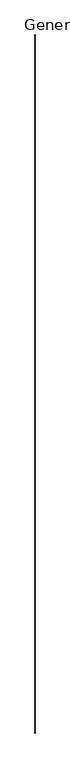
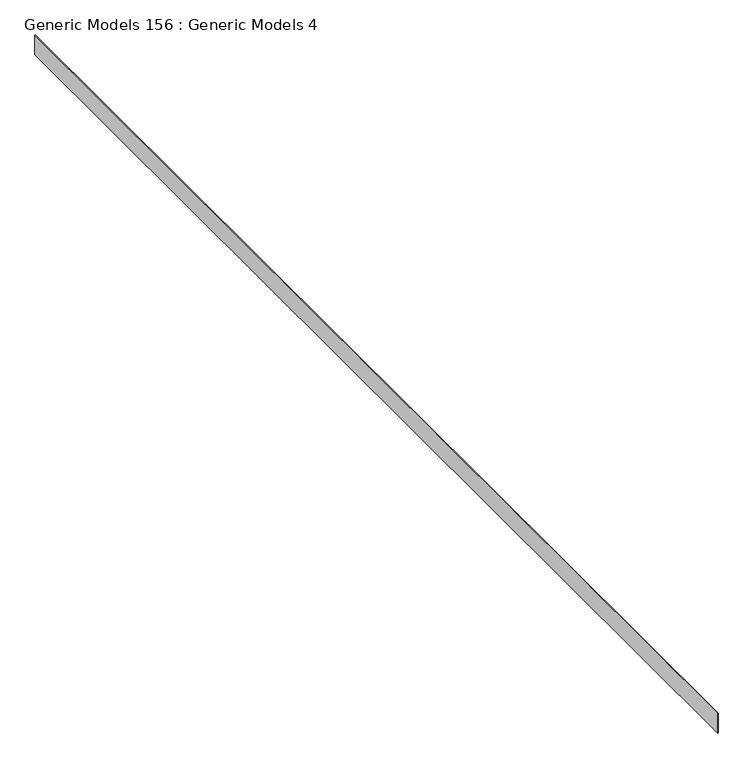
"""IFC4 building model written with IfcOpenShell, lengths in millimetres: proxy geometry, Generic Models 156 : Generic Models 4."""

from ifc_helpers import new_model, si_unit, frame, origin, place, context, project, spatial, polyline, outline, extrude, source, transform, mapped, element, save


def generic_models_156_generic_models_4_3786cacd(model_context):
    return source(origin(), model_context, "Body", "SweptSolid", [
        extrude(outline(polyline([(-10232.9347239, -5493.3230338), (-10236.1097239, -5493.3230338), (-10236.1097239, 7054.2769662), (-10232.9347239, 7054.2769662), (-10232.9347239, -5493.3230338)])), frame((0.0, 0.0, 122573.1444509), z_axis=(0.0, 0.0, 1.0), x_axis=(1.0, 0.0, 0.0)), (0.0, 0.0, 1.0), 220.5790364),
    ])


if __name__ == "__main__":
    model = new_model("IFC4")
    model_context = context("Model", 3, world=origin())
    ifc_project = project(units=[si_unit("LENGTHUNIT", "METRE", prefix="MILLI")], contexts=[model_context])
    site = spatial("IfcSite", under=ifc_project)
    building = spatial("IfcBuilding", under=site)
    placement = place(None, origin())
    generic_models_156_generic_models_4_shape = generic_models_156_generic_models_4_3786cacd(model_context)
    element("IfcBuildingElementProxy", 1, Name="Generic Models 156 : Generic Models 4", ObjectType="Generic Models 156 : Generic Models 4", at=placement, inside=building, context=model_context, shape_type="MappedRepresentation", body=[
        mapped(generic_models_156_generic_models_4_shape, transform((0.0, 0.0, 0.0), x_axis=(1.0, 0.0, 0.0), y_axis=(0.0, 1.0, 0.0), z_axis=(0.0, 0.0, 1.0))),
    ])
    save(model, "model.ifc")

# Revit data of these elements
# Element 1 (IfcBuildingElementProxy, "Generic Models 156 : Generic Models 4")
#   Materials on its faces: "_MORTAR SCRATCH COAT"
# Materials
#   "_MORTAR SCRATCH COAT": class "Generic", colour RGB 233 233 233, transparency 0, Cost = 0
